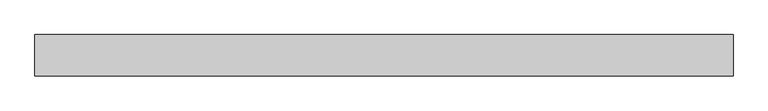
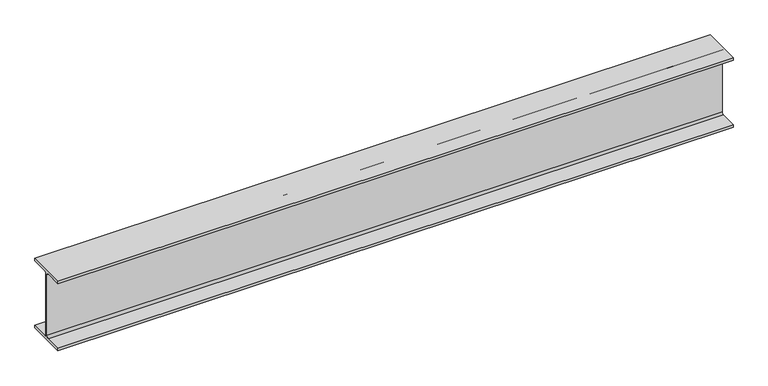
"""IFC4 building model written with IfcOpenShell, lengths in millimetres: beam geometry, Old_Steel Beam_H-KSD3502 : H_SB_ASB_H-250×125x6x9."""

from ifc_helpers import new_model, si_unit, point, frame, frame_2d, origin, place, context, project, spatial, polyline, circle_curve, trimmed, segment, composite_curve, outline, extrude, source, transform, mapped, element, save


def beam_b704906e(model_context):
    return source(origin(), model_context, "Body", "SweptSolid", [
        extrude(outline(composite_curve([segment(polyline([(82.5, -141.5), (82.5, -151.7), (-82.5, -151.7), (-82.5, -141.5), (-11.9, -141.5)]), True, "CONTINUOUS"), segment(trimmed(circle_curve(frame_2d((-11.9, -132.6)), 8.9), [point((-11.9, -141.5))], [point((-3.0, -132.6))], True, "CARTESIAN"), True, "CONTINUOUS"), segment(polyline([(-3.0, -132.6), (-3.0, 132.6)]), True, "CONTINUOUS"), segment(trimmed(circle_curve(frame_2d((-11.9, 132.6)), 8.9), [point((-3.0, 132.6))], [point((-11.9, 141.5))], True, "CARTESIAN"), True, "CONTINUOUS"), segment(polyline([(-11.9, 141.5), (-82.5, 141.5), (-82.5, 151.7), (82.5, 151.7), (82.5, 141.5), (11.9, 141.5)]), True, "CONTINUOUS"), segment(trimmed(circle_curve(frame_2d((11.9, 132.6)), 8.9), [point((11.9, 141.5))], [point((3.0, 132.6))], True, "CARTESIAN"), True, "CONTINUOUS"), segment(polyline([(3.0, 132.6), (3.0, -132.6)]), True, "CONTINUOUS"), segment(trimmed(circle_curve(frame_2d((11.9, -132.6)), 8.9), [point((3.0, -132.6))], [point((11.9, -141.5))], True, "CARTESIAN"), True, "CONTINUOUS"), segment(polyline([(11.9, -141.5), (82.5, -141.5)]), True, "CONTINUOUS")], self_intersect=False)), frame((-1382.298157, 0.0, 0.0), z_axis=(1.0, 0.0, 0.0), x_axis=(0.0, 1.0, 0.0)), (0.0, 0.0, 1.0), 2794.5982),
    ])


if __name__ == "__main__":
    model = new_model("IFC4")
    model_context = context("Model", 3, world=origin())
    ifc_project = project(units=[si_unit("LENGTHUNIT", "METRE", prefix="MILLI")], contexts=[model_context])
    site = spatial("IfcSite", under=ifc_project)
    building = spatial("IfcBuilding", under=site)
    placement = place(None, origin())
    beam_shape = beam_b704906e(model_context)
    element("IfcBeam", 1, ObjectType="Old_Steel Beam_H-KSD3502 : H_SB_ASB_H-250×125x6x9", at=placement, inside=building, context=model_context, shape_type="MappedRepresentation", body=[
        mapped(beam_shape, transform((0.0, 0.0, 0.0), x_axis=(1.0, 0.0, 0.0), y_axis=(0.0, 1.0, 0.0), z_axis=(0.0, 0.0, 1.0))),
    ])
    save(model, "model.ifc")

# Revit data of these elements
# Type "Old_Steel Beam_H-KSD3502 : H_SB_ASB_H-250×125x6x9"
#   Width = 12.5 cm
#   Web Thickness = 0.6 cm
#   Web Fillet = 1.2 cm
#   Warping Constant = 42539.8 cm⁶
#   Torsional Moment of Inertia = 7.8102 cm⁴
#   Torsional Modulus = 1.0 cm³
#   Section Area = 37.66 cm²
#   Plastic Modulus weak axis = 73.1 cm³
#   Plastic Modulus strong axis = 366.0 cm³
#   Perimeter = 0.97 m²/m
#   Nominal Weight = 29.60 kgf/m
#   Moment of Inertia weak axis = 294.00 cm⁴
#   Moment of Inertia strong axis = 4050.00 cm⁴
#   Height = 25.0 cm
#   Flange Thickness = 0.9 cm
#   Elastic Modulus weak axis = 47.0 cm³
#   Elastic Modulus strong axis = 324.0 cm³
#   Centroid Vertical = 12.5 cm
#   Centroid Horizontal = 6.25 cm
#   Length [instance default] = 1.5240 m
#   Structural Material [instance default] = Steel, 45-345
#   Assembly Code = ""
# Element 1 (IfcBeam, "Old_Steel Beam_H-KSD3502 : H_SB_ASB_H-250×125x6x9")
#   Structural Material = none
# Materials
#   "Steel, 45-345": class "Metal", colour RGB 189 187 185, transparency 0, Description = "Steel 345 MPa", Cost = 0
